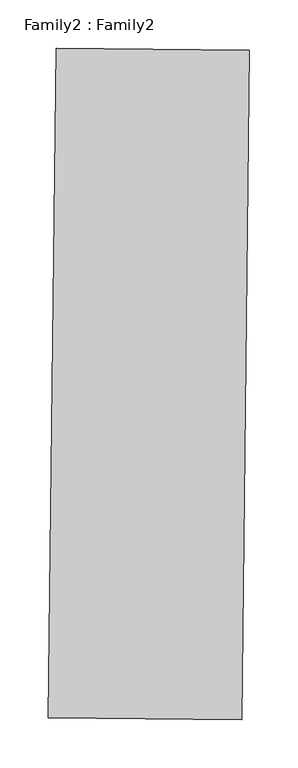
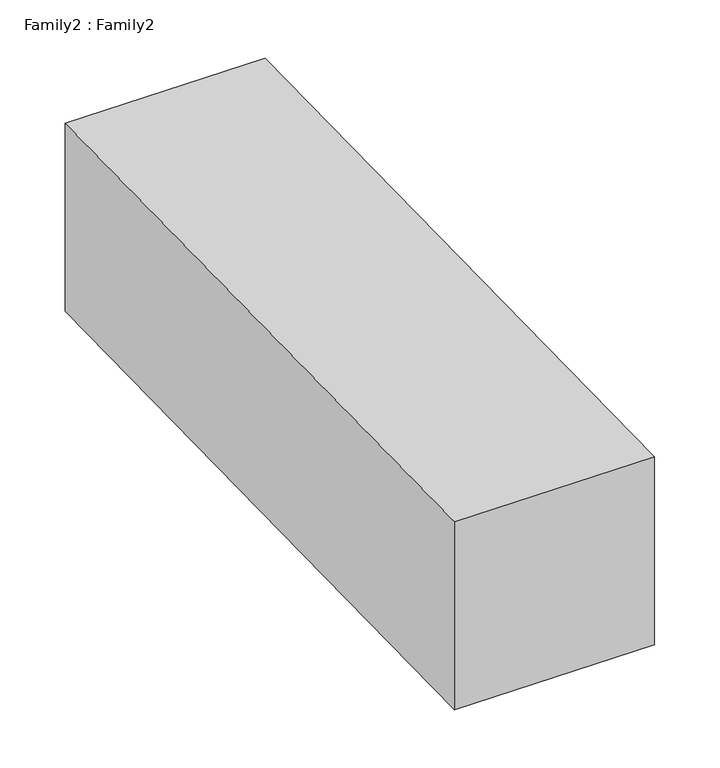
"""IFC4 building model written with IfcOpenShell, lengths in millimetres: proxy geometry, Family2 : Family2."""

from ifc_helpers import new_model, si_unit, origin, place, context, project, spatial, faceted_brep, source, transform, mapped, element, save


def family2_family2_390b1421(model_context):
    return source(origin(), model_context, "Body", "Brep", [
        faceted_brep([(-3947.4886476, -6420.3281868, 1.0945136), (-3947.4886476, -6420.3281868, 201.0945136), (-3939.3541469, -5727.2719358, 202.060409), (-3939.3541469, -5727.2719358, 2.060409), (-3747.4974576, -6422.2053995, 201.0945136), (-3739.3629569, -5729.1491484, 202.060409), (-3747.4974576, -6422.2053995, 1.0945136), (-3739.3629569, -5729.1491484, 2.060409)], [[[0, 1, 2, 3]], [[1, 4, 5, 2]], [[4, 6, 7, 5]], [[6, 0, 3, 7]], [[3, 2, 5, 7]], [[0, 6, 4, 1]]]),
    ])


if __name__ == "__main__":
    model = new_model("IFC4")
    model_context = context("Model", 3, world=origin())
    ifc_project = project(units=[si_unit("LENGTHUNIT", "METRE", prefix="MILLI")], contexts=[model_context])
    site = spatial("IfcSite", under=ifc_project)
    building = spatial("IfcBuilding", under=site)
    placement = place(None, origin())
    family2_family2_shape = family2_family2_390b1421(model_context)
    element("IfcBuildingElementProxy", 1, Name="Family2 : Family2", ObjectType="Family2 : Family2", at=placement, inside=building, context=model_context, shape_type="MappedRepresentation", body=[
        mapped(family2_family2_shape, transform((0.0, 0.0, 0.0), x_axis=(1.0, 0.0, 0.0), y_axis=(0.0, 1.0, 0.0), z_axis=(0.0, 0.0, 1.0))),
    ])
    save(model, "model.ifc")

# Revit data of these elements
# Type "Family2 : Family2"
#   Default Elevation = 0
